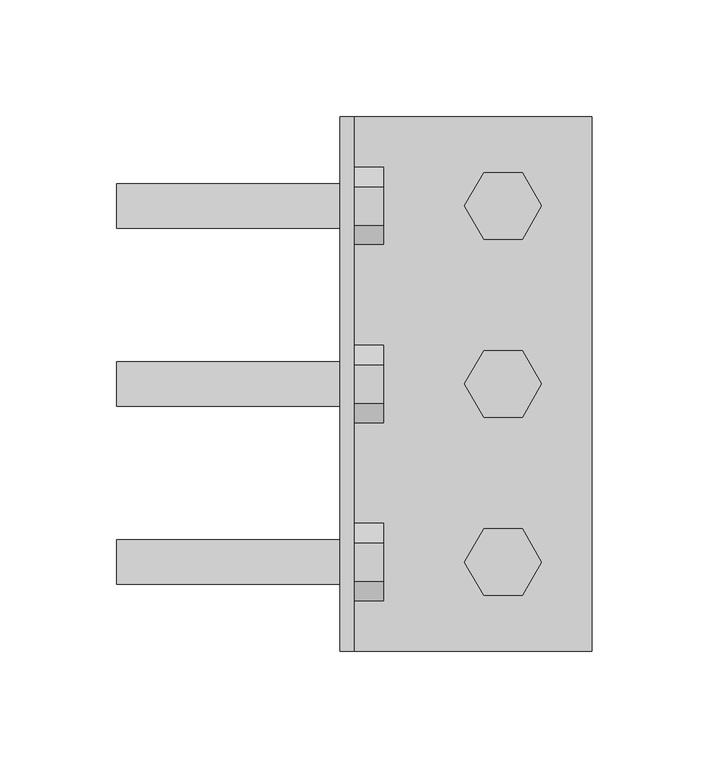
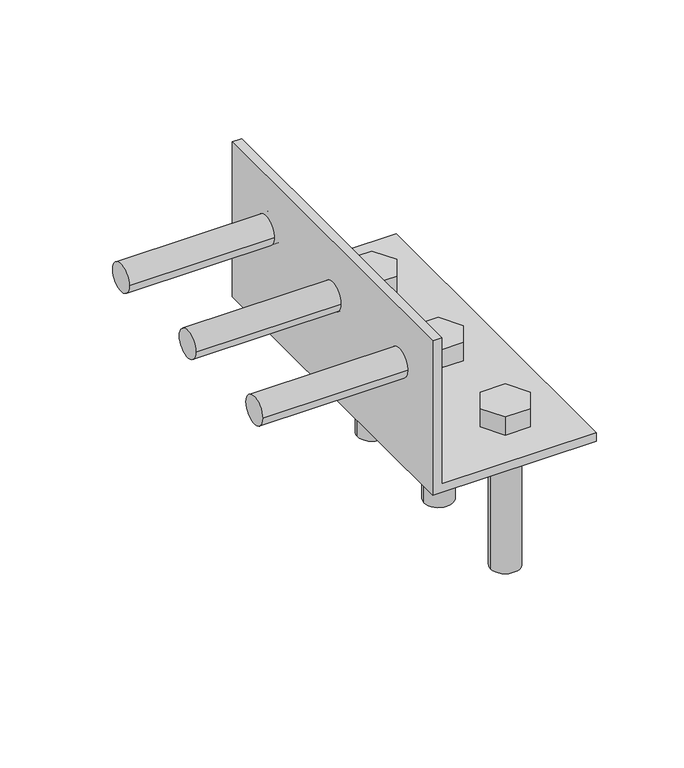
"""IFC4 building model written with IfcOpenShell, lengths in millimetres: fastener geometry, SIMPSON - HLPC/HLGPC Heavy Angles and Gussets : SIMPSON -HL49 - 9 X 4.25 - .75 Bolt - HDG."""

from ifc_helpers import new_model, si_unit, point, frame, frame_2d, origin, place, context, project, spatial, polyline, circle_curve, trimmed, segment, composite_curve, outline, extrude, source, transform, mapped, element, save
from ifc_brep_helpers import plane_surface, revolved_surface, advanced_brep


def fastener_bc8651eb(model_context):
    return source(origin(), model_context, "Body", "SolidModel", [
        extrude(outline(composite_curve([segment(trimmed(circle_curve(frame_2d((-76.2, 69.85)), 9.525), [point((-85.725, 69.85))], [point((-66.675, 69.85))], False, "CARTESIAN"), True, "CONTINUOUS"), segment(trimmed(circle_curve(frame_2d((-76.2, 69.85)), 9.525), [point((-66.675, 69.85))], [point((-85.725, 69.85))], False, "CARTESIAN"), True, "CONTINUOUS")], self_intersect=False)), frame((-95.5476562, 0.0, 0.0), z_axis=(1.0, 0.0, 0.0), x_axis=(0.0, 1.0, 0.0)), (0.0, 0.0, 1.0), 101.6),
        extrude(outline(polyline([(-92.6977839, 69.85), (-84.448892, 84.1375), (-67.951108, 84.1375), (-59.7022161, 69.85), (-67.951108, 55.5625), (-84.448892, 55.5625), (-92.6977839, 69.85)])), frame((6.0523438, 0.0, 0.0), z_axis=(1.0, 0.0, 0.0), x_axis=(0.0, 1.0, 0.0)), (0.0, 0.0, 1.0), 12.7),
        extrude(outline(composite_curve([segment(trimmed(circle_curve(frame_2d((0.0, 69.85)), 9.525), [point((-9.525, 69.85))], [point((9.525, 69.85))], False, "CARTESIAN"), True, "CONTINUOUS"), segment(trimmed(circle_curve(frame_2d((0.0, 69.85)), 9.525), [point((9.525, 69.85))], [point((-9.525, 69.85))], False, "CARTESIAN"), True, "CONTINUOUS")], self_intersect=False)), frame((-95.5476562, 0.0, 0.0), z_axis=(1.0, 0.0, 0.0), x_axis=(0.0, 1.0, 0.0)), (0.0, 0.0, 1.0), 101.6),
        extrude(outline(polyline([(-16.4977839, 69.85), (-8.248892, 84.1375), (8.248892, 84.1375), (16.4977839, 69.85), (8.248892, 55.5625), (-8.248892, 55.5625), (-16.4977839, 69.85)])), frame((6.0523438, 0.0, 0.0), z_axis=(1.0, 0.0, 0.0), x_axis=(0.0, 1.0, 0.0)), (0.0, 0.0, 1.0), 12.7),
        extrude(outline(composite_curve([segment(trimmed(circle_curve(frame_2d((76.2, 69.85)), 9.525), [point((66.675, 69.85))], [point((85.725, 69.85))], False, "CARTESIAN"), True, "CONTINUOUS"), segment(trimmed(circle_curve(frame_2d((76.2, 69.85)), 9.525), [point((85.725, 69.85))], [point((66.675, 69.85))], False, "CARTESIAN"), True, "CONTINUOUS")], self_intersect=False)), frame((-95.5476562, 0.0, 0.0), z_axis=(1.0, 0.0, 0.0), x_axis=(0.0, 1.0, 0.0)), (0.0, 0.0, 1.0), 101.6),
        extrude(outline(polyline([(59.7022161, 69.85), (67.951108, 84.1375), (84.448892, 84.1375), (92.6977839, 69.85), (84.448892, 55.5625), (67.951108, 55.5625), (59.7022161, 69.85)])), frame((6.0523438, 0.0, 0.0), z_axis=(1.0, 0.0, 0.0), x_axis=(0.0, 1.0, 0.0)), (0.0, 0.0, 1.0), 12.7),
        extrude(outline(composite_curve([segment(trimmed(circle_curve(frame_2d((69.85, 76.2)), 9.525), [point((60.325, 76.2))], [point((79.375, 76.2))], False, "CARTESIAN"), True, "CONTINUOUS"), segment(trimmed(circle_curve(frame_2d((69.85, 76.2)), 9.525), [point((79.375, 76.2))], [point((60.325, 76.2))], False, "CARTESIAN"), True, "CONTINUOUS")], self_intersect=False)), frame((0.0, 0.0, -95.5476563), z_axis=(0.0, 0.0, 1.0), x_axis=(1.0, 0.0, 0.0)), (0.0, 0.0, 1.0), 101.6),
        extrude(outline(polyline([(53.3522161, 76.2), (61.601108, 90.4875), (78.098892, 90.4875), (86.3477839, 76.2), (78.098892, 61.9125), (61.601108, 61.9125), (53.3522161, 76.2)])), frame((0.0, 0.0, 6.0523437), z_axis=(0.0, 0.0, 1.0), x_axis=(1.0, 0.0, 0.0)), (0.0, 0.0, 1.0), 12.7),
        extrude(outline(composite_curve([segment(trimmed(circle_curve(frame_2d((69.85, 0.0)), 9.525), [point((60.325, 0.0))], [point((79.375, 0.0))], False, "CARTESIAN"), True, "CONTINUOUS"), segment(trimmed(circle_curve(frame_2d((69.85, 0.0)), 9.525), [point((79.375, 0.0))], [point((60.325, 0.0))], False, "CARTESIAN"), True, "CONTINUOUS")], self_intersect=False)), frame((0.0, 0.0, -95.5476563), z_axis=(0.0, 0.0, 1.0), x_axis=(1.0, 0.0, 0.0)), (0.0, 0.0, 1.0), 101.6),
        extrude(outline(polyline([(53.3522161, 0.0), (61.601108, 14.2875), (78.098892, 14.2875), (86.3477839, 0.0), (78.098892, -14.2875), (61.601108, -14.2875), (53.3522161, 0.0)])), frame((0.0, 0.0, 6.0523437), z_axis=(0.0, 0.0, 1.0), x_axis=(1.0, 0.0, 0.0)), (0.0, 0.0, 1.0), 12.7),
        extrude(outline(composite_curve([segment(trimmed(circle_curve(frame_2d((69.85, -76.2)), 9.525), [point((60.325, -76.2))], [point((79.375, -76.2))], False, "CARTESIAN"), True, "CONTINUOUS"), segment(trimmed(circle_curve(frame_2d((69.85, -76.2)), 9.525), [point((79.375, -76.2))], [point((60.325, -76.2))], False, "CARTESIAN"), True, "CONTINUOUS")], self_intersect=False)), frame((0.0, 0.0, -95.5476563), z_axis=(0.0, 0.0, 1.0), x_axis=(1.0, 0.0, 0.0)), (0.0, 0.0, 1.0), 101.6),
        extrude(outline(polyline([(53.3522161, -76.2), (61.601108, -61.9125), (78.098892, -61.9125), (86.3477839, -76.2), (78.098892, -90.4875), (61.601108, -90.4875), (53.3522161, -76.2)])), frame((0.0, 0.0, 6.0523437), z_axis=(0.0, 0.0, 1.0), x_axis=(1.0, 0.0, 0.0)), (0.0, 0.0, 1.0), 12.7),
        advanced_brep(
        [(6.0523438, 114.3, 107.95), (6.0523438, -114.3, 107.95), (6.0523438, -114.3, 6.0523437), (6.0523438, 114.3, 6.0523437), (6.0523438, -66.675, 69.85), (6.0523438, -85.725, 69.85), (6.0523438, 9.525, 69.85), (6.0523438, -9.525, 69.85), (6.0523438, 85.725, 69.85), (6.0523438, 66.675, 69.85), (0.0, -114.3, 107.95), (0.0, 114.3, 107.95), (0.0, 114.3, 0.0), (0.0, -114.3, 0.0), (0.0, -85.725, 69.85), (0.0, -66.675, 69.85), (0.0, -9.525, 69.85), (0.0, 9.525, 69.85), (0.0, 66.675, 69.85), (0.0, 85.725, 69.85), (107.95, -114.3, 0.0), (107.95, -114.3, 6.0523437), (107.95, 114.3, 6.0523437), (107.95, 114.3, 0.0), (79.375, -76.2, 6.0523437), (60.325, -76.2, 6.0523437), (79.375, 0.0, 6.0523437), (60.325, 0.0, 6.0523437), (79.375, 76.2, 6.0523437), (60.325, 76.2, 6.0523437), (60.325, -76.2, 0.0), (79.375, -76.2, 0.0), (60.325, 0.0, 0.0), (79.375, 0.0, 0.0), (60.325, 76.2, 0.0), (79.375, 76.2, 0.0)],
        [
            (0, 1),
            (1, 2),
            (2, 3),
            (3, 0),
            (4, 5, circle_curve(frame((6.0523438, -76.2, 69.85), z_axis=(-1.0, 0.0, 0.0), x_axis=(0.0, 1.0, 0.0)), 9.525)),
            (5, 4, circle_curve(frame((6.0523438, -76.2, 69.85), z_axis=(-1.0, 0.0, 0.0), x_axis=(0.0, 1.0, 0.0)), 9.525)),
            (6, 7, circle_curve(frame((6.0523438, 0.0, 69.85), z_axis=(-1.0, 0.0, 0.0), x_axis=(0.0, 1.0, 0.0)), 9.525)),
            (7, 6, circle_curve(frame((6.0523438, 0.0, 69.85), z_axis=(-1.0, 0.0, 0.0), x_axis=(0.0, 1.0, 0.0)), 9.525)),
            (8, 9, circle_curve(frame((6.0523438, 76.2, 69.85), z_axis=(-1.0, 0.0, 0.0), x_axis=(0.0, 1.0, 0.0)), 9.525)),
            (9, 8, circle_curve(frame((6.0523438, 76.2, 69.85), z_axis=(-1.0, 0.0, 0.0), x_axis=(0.0, 1.0, 0.0)), 9.525)),
            (10, 11),
            (11, 12),
            (12, 13),
            (13, 10),
            (14, 15, circle_curve(frame((0.0, -76.2, 69.85), z_axis=(1.0, 0.0, 0.0), x_axis=(0.0, 1.0, 0.0)), 9.525)),
            (15, 14, circle_curve(frame((0.0, -76.2, 69.85), z_axis=(1.0, 0.0, 0.0), x_axis=(0.0, 1.0, 0.0)), 9.525)),
            (16, 17, circle_curve(frame((0.0, 0.0, 69.85), z_axis=(1.0, 0.0, 0.0), x_axis=(0.0, 1.0, 0.0)), 9.525)),
            (17, 16, circle_curve(frame((0.0, 0.0, 69.85), z_axis=(1.0, 0.0, 0.0), x_axis=(0.0, 1.0, 0.0)), 9.525)),
            (18, 19, circle_curve(frame((0.0, 76.2, 69.85), z_axis=(1.0, 0.0, 0.0), x_axis=(0.0, 1.0, 0.0)), 9.525)),
            (19, 18, circle_curve(frame((0.0, 76.2, 69.85), z_axis=(1.0, 0.0, 0.0), x_axis=(0.0, 1.0, 0.0)), 9.525)),
            (0, 11),
            (10, 1),
            (13, 20),
            (20, 21),
            (21, 2),
            (3, 22),
            (22, 23),
            (23, 12),
            (21, 22),
            (24, 25, circle_curve(frame((69.85, -76.2, 6.0523437), z_axis=(0.0, 0.0, -1.0), x_axis=(1.0, 0.0, 0.0)), 9.525)),
            (25, 24, circle_curve(frame((69.85, -76.2, 6.0523437), z_axis=(0.0, 0.0, -1.0), x_axis=(1.0, 0.0, 0.0)), 9.525)),
            (26, 27, circle_curve(frame((69.85, 0.0, 6.0523437), z_axis=(0.0, 0.0, -1.0), x_axis=(1.0, 0.0, 0.0)), 9.525)),
            (27, 26, circle_curve(frame((69.85, 0.0, 6.0523437), z_axis=(0.0, 0.0, -1.0), x_axis=(1.0, 0.0, 0.0)), 9.525)),
            (28, 29, circle_curve(frame((69.85, 76.2, 6.0523437), z_axis=(0.0, 0.0, -1.0), x_axis=(1.0, 0.0, 0.0)), 9.525)),
            (29, 28, circle_curve(frame((69.85, 76.2, 6.0523437), z_axis=(0.0, 0.0, -1.0), x_axis=(1.0, 0.0, 0.0)), 9.525)),
            (23, 20),
            (30, 31, circle_curve(frame((69.85, -76.2, 0.0), z_axis=(0.0, 0.0, 1.0), x_axis=(1.0, 0.0, 0.0)), 9.525)),
            (31, 30, circle_curve(frame((69.85, -76.2, 0.0), z_axis=(0.0, 0.0, 1.0), x_axis=(1.0, 0.0, 0.0)), 9.525)),
            (32, 33, circle_curve(frame((69.85, 0.0, 0.0), z_axis=(0.0, 0.0, 1.0), x_axis=(1.0, 0.0, 0.0)), 9.525)),
            (33, 32, circle_curve(frame((69.85, 0.0, 0.0), z_axis=(0.0, 0.0, 1.0), x_axis=(1.0, 0.0, 0.0)), 9.525)),
            (34, 35, circle_curve(frame((69.85, 76.2, 0.0), z_axis=(0.0, 0.0, 1.0), x_axis=(1.0, 0.0, 0.0)), 9.525)),
            (35, 34, circle_curve(frame((69.85, 76.2, 0.0), z_axis=(0.0, 0.0, 1.0), x_axis=(1.0, 0.0, 0.0)), 9.525)),
            (24, 31),
            (30, 25),
            (26, 33),
            (32, 27),
            (28, 35),
            (34, 29),
            (4, 15),
            (14, 5),
            (6, 17),
            (16, 7),
            (8, 19),
            (18, 9),
        ],
        [
            plane_surface(frame((6.0523438, -114.3, 107.95), z_axis=(1.0, 0.0, 0.0), x_axis=(0.0, -1.0, 0.0))),
            plane_surface(frame((0.0, -114.3, 107.95), z_axis=(-1.0, 0.0, 0.0), x_axis=(0.0, 1.0, 0.0))),
            plane_surface(frame((6.0523438, 114.3, 107.95), z_axis=(0.0, 0.0, 1.0), x_axis=(-1.0, 0.0, 0.0))),
            plane_surface(frame((6.0523438, -114.3, 107.95), z_axis=(0.0, -1.0, 0.0), x_axis=(-1.0, 0.0, 0.0))),
            plane_surface(frame((6.0523438, 114.3, 6.0523437), z_axis=(0.0, 1.0, 0.0), x_axis=(-1.0, 0.0, 0.0))),
            plane_surface(frame((0.0, 114.3, 6.0523437), z_axis=(0.0, 0.0, 1.0), x_axis=(-1.0, 0.0, 0.0))),
            plane_surface(frame((0.0, 114.3, 0.0), z_axis=(0.0, 0.0, -1.0), x_axis=(1.0, 0.0, 0.0))),
            plane_surface(frame((107.95, -114.3, 6.0523437), z_axis=(1.0, 0.0, 0.0), x_axis=(0.0, 0.0, -1.0))),
            revolved_surface(polyline([(79.375, -76.2, 6.0523437), (79.375, -76.2, 0.0)]), (69.85, -76.2, 0.0), (0.0, 0.0, 1.0)),
            revolved_surface(polyline([(79.375, 0.0, 6.0523437), (79.375, 0.0, 0.0)]), (69.85, 0.0, 0.0), (0.0, 0.0, 1.0)),
            revolved_surface(polyline([(79.375, 76.2, 6.0523437), (79.375, 76.2, 0.0)]), (69.85, 76.2, 0.0), (0.0, 0.0, 1.0)),
            revolved_surface(polyline([(6.0523438, -66.675, 69.85), (0.0, -66.675, 69.85)]), (0.0, -76.2, 69.85), (1.0, 0.0, 0.0)),
            revolved_surface(polyline([(6.0523438, 9.525, 69.85), (0.0, 9.525, 69.85)]), (0.0, 0.0, 69.85), (1.0, 0.0, 0.0)),
            revolved_surface(polyline([(6.0523438, 85.72500000000001, 69.85), (0.0, 85.72500000000001, 69.85)]), (0.0, 76.2, 69.85), (1.0, 0.0, 0.0)),
        ],
        [
            (0, [[1, 2, 3, 4], [5, 6], [7, 8], [9, 10]]),
            (1, [[11, 12, 13, 14], [15, 16], [17, 18], [19, 20]]),
            (2, [[-1, 21, -11, 22]]),
            (3, [[-2, -22, -14, 23, 24, 25]]),
            (4, [[-4, 26, 27, 28, -12, -21]]),
            (5, [[29, -26, -3, -25], [30, 31], [32, 33], [34, 35]]),
            (6, [[36, -23, -13, -28], [37, 38], [39, 40], [41, 42]]),
            (7, [[-29, -24, -36, -27]]),
            (8, [[43, -37, 44, -30]]),
            (8, [[-43, -31, -44, -38]]),
            (9, [[45, -39, 46, -32]]),
            (9, [[-45, -33, -46, -40]]),
            (10, [[47, -41, 48, -34]]),
            (10, [[-47, -35, -48, -42]]),
            (11, [[49, -15, 50, -5]]),
            (11, [[-49, -6, -50, -16]]),
            (12, [[51, -17, 52, -7]]),
            (12, [[-51, -8, -52, -18]]),
            (13, [[53, -19, 54, -9]]),
            (13, [[-53, -10, -54, -20]]),
        ],
    ),
    ])


if __name__ == "__main__":
    model = new_model("IFC4")
    model_context = context("Model", 3, world=origin())
    ifc_project = project(units=[si_unit("LENGTHUNIT", "METRE", prefix="MILLI")], contexts=[model_context])
    site = spatial("IfcSite", under=ifc_project)
    building = spatial("IfcBuilding", under=site)
    placement = place(None, origin())
    fastener_shape = fastener_bc8651eb(model_context)
    element("IfcFastener", 1, ObjectType="SIMPSON - HLPC/HLGPC Heavy Angles and Gussets : SIMPSON -HL49 - 9 X 4.25 - .75 Bolt - HDG", at=placement, inside=building, context=model_context, shape_type="MappedRepresentation", body=[
        mapped(fastener_shape, transform((0.0, 0.0, 0.0), x_axis=(1.0, 0.0, 0.0), y_axis=(0.0, 1.0, 0.0), z_axis=(0.0, 0.0, 1.0))),
    ])
    save(model, "model.ifc")

# Revit data of these elements
# Type "SIMPSON - HLPC/HLGPC Heavy Angles and Gussets : SIMPSON -HL49 - 9 X 4.25 - .75 Bolt - HDG"
#   URL = "https://www.strongtie.com/classiccollection_architecturalproductsgroup/hlpc-hlgpc_productgroup_wcc/p/hlpc.hlgpc"
#   L = 0' - 9"
#   Hole Radius = 0' - 0 3/8"
#   D4 = 0' - 5"
#   D2 = 0' - 3"
#   D1 = 0' - 1 1/2"
#   D3 = 0' - 2 3/4"
#   Ga. = 0' - 0 61/256"
#   W1 & W2 = 0' - 4 1/4"
#   Default Elevation = 4' - 0"
#   Bolt Visibility - 3B = no
#   Bolt Visibility - 3A = yes
#   Bolt Visibility - 2B = no
#   Bolt Visibility - 2A = yes
#   Bolt Visibility - 1B = no
#   Bolt Visibility - 1A = yes
#   Bolt Visibility = yes
#   Bolt Size = element 1298415
# Element 1 (IfcFastener, "SIMPSON - HLPC/HLGPC Heavy Angles and Gussets : SIMPSON -HL49 - 9 X 4.25 - .75 Bolt - HDG")
#   Materials on its faces: "1\" GALV. LAG BOLT (LENGTH = 1/2\" SHY OF GLULAM DEPTH) -  (GALV. THRU BOLT IF PLATE ON OPP. SIDE OF STRUCT MEMBER)"
# Materials
#   "1\" GALV. LAG BOLT (LENGTH = 1/2\" SHY OF GLULAM DEPTH) -  (GALV. THRU BOLT IF PLATE ON OPP. SIDE OF STRUCT MEMBER)": class "Generic", colour RGB 120 120 120, transparency 0, Cost = 0
